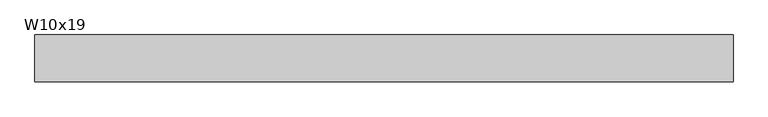
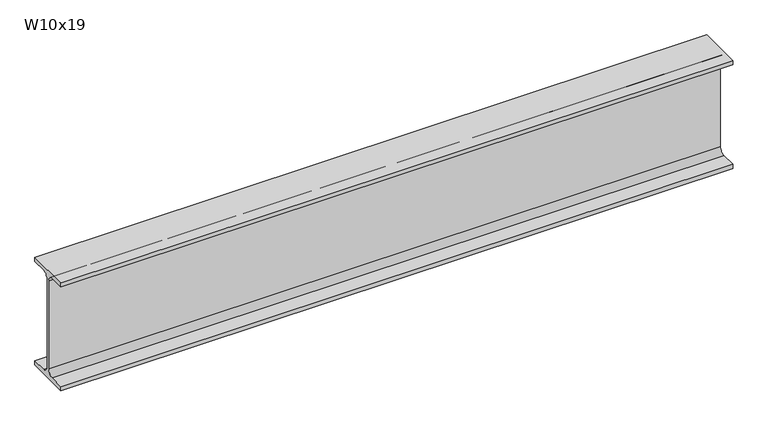
"""IFC4 building model written with IfcOpenShell, lengths in millimetres: beam geometry, RME W-Wide Flange : W10x19."""

from ifc_helpers import new_model, si_unit, point, frame, frame_2d, origin, place, context, project, spatial, polyline, circle_curve, trimmed, segment, composite_curve, outline, extrude, source, transform, mapped, element, save


def w10x19_6ecbe7fb(model_context):
    return source(origin(), model_context, "Body", "SweptSolid", [
        extrude(outline(composite_curve([segment(polyline([(51.054, -119.507), (51.054, -129.54), (-51.054, -129.54), (-51.054, -119.507), (-16.9545, -119.507)]), True, "CONTINUOUS"), segment(trimmed(circle_curve(frame_2d((-16.9545, -105.7275)), 13.7795), [point((-16.9545, -119.507))], [point((-3.175, -105.7275))], True, "CARTESIAN"), True, "CONTINUOUS"), segment(polyline([(-3.175, -105.7275), (-3.175, 105.7275)]), True, "CONTINUOUS"), segment(trimmed(circle_curve(frame_2d((-16.9545, 105.7275)), 13.7795), [point((-3.175, 105.7275))], [point((-16.9545, 119.507))], True, "CARTESIAN"), True, "CONTINUOUS"), segment(polyline([(-16.9545, 119.507), (-51.054, 119.507), (-51.054, 129.54), (51.054, 129.54), (51.054, 119.507), (16.9545, 119.507)]), True, "CONTINUOUS"), segment(trimmed(circle_curve(frame_2d((16.9545, 105.7275)), 13.7795), [point((16.9545, 119.507))], [point((3.175, 105.7275))], True, "CARTESIAN"), True, "CONTINUOUS"), segment(polyline([(3.175, 105.7275), (3.175, -105.7275)]), True, "CONTINUOUS"), segment(trimmed(circle_curve(frame_2d((16.9545, -105.7275)), 13.7795), [point((3.175, -105.7275))], [point((16.9545, -119.507))], True, "CARTESIAN"), True, "CONTINUOUS"), segment(polyline([(16.9545, -119.507), (51.054, -119.507)]), True, "CONTINUOUS")], self_intersect=False)), frame((-763.4165055, 0.0, 0.0), z_axis=(1.0, 0.0, 0.0), x_axis=(0.0, 1.0, 0.0)), (0.0, 0.0, 1.0), 1526.8330109),
    ])


if __name__ == "__main__":
    model = new_model("IFC4")
    model_context = context("Model", 3, world=origin())
    ifc_project = project(units=[si_unit("LENGTHUNIT", "METRE", prefix="MILLI")], contexts=[model_context])
    site = spatial("IfcSite", under=ifc_project)
    building = spatial("IfcBuilding", under=site)
    placement = place(None, origin())
    w10x19_shape = w10x19_6ecbe7fb(model_context)
    element("IfcBeam", 1, ObjectType="RME W-Wide Flange : W10x19", at=placement, inside=building, context=model_context, shape_type="MappedRepresentation", body=[
        mapped(w10x19_shape, transform((0.0, 0.0, 0.0), x_axis=(1.0, 0.0, 0.0), y_axis=(0.0, 1.0, 0.0), z_axis=(0.0, 0.0, 1.0))),
    ])
    save(model, "model.ifc")

# Revit data of these elements
# Type "RME W-Wide Flange : W10x19"
#   WELD P [instance default] = ""
#   WELD LE [instance default] = ""
#   WELD D [instance default] = ""
#   TOP SECTION SIZE [instance default] = ""
#   TOP SECTION LENGTH [instance default] = ""
#   REMARKS [instance default] = ""
#   REINF TYPE [instance default] = ""
#   Nominal Size = "W24"
#   End Bearing Capacity [instance default] = ""
#   BOT SECTION SIZE [instance default] = ""
#   BOT SECTION LENGTH [instance default] = ""
#   Assembly Code = "B10"
#   W = 19
#   Start Extension Calculation [instance default] = 10' - 0"
#   Start Extension [instance default] = -0' - 0 1/2"
#   End Extension Calculation [instance default] = 10' - 0"
#   End Extension [instance default] = -0' - 0 1/2"
#   Length [instance default] = 5' - 0"
#   bf = 0' - 4.02"
#   d = 0' - 10.2"
#   k = 0' - 0 15/16"
#   k2 = 0' - 0.5425"
#   tf = 0' - 0.395"
#   tw = 0' - 0 1/4"
#   A = 0.0390278 SF
#   Structural Material [instance default] = Metal - Steel - ASTM A992
# Element 1 (IfcBeam, "RME W-Wide Flange : W10x19")
#   Length = 5' - 0.11154"
#   Materials on its faces: "Metal - Steel - ASTM A992"
# Materials
#   "Metal - Steel - ASTM A992": class "Metal", colour RGB 255 128 0, transparency 0
